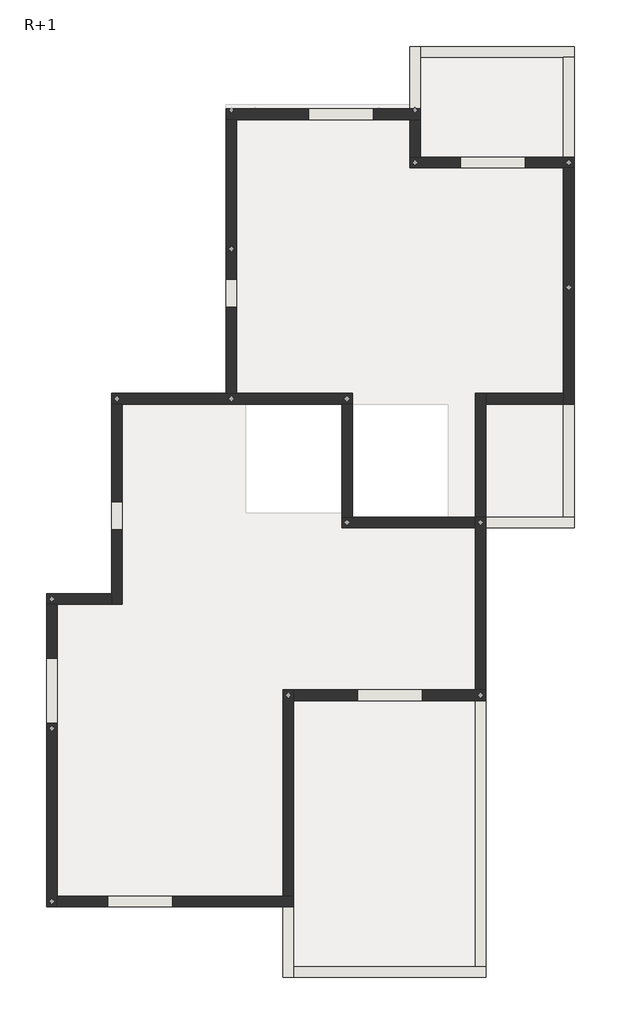
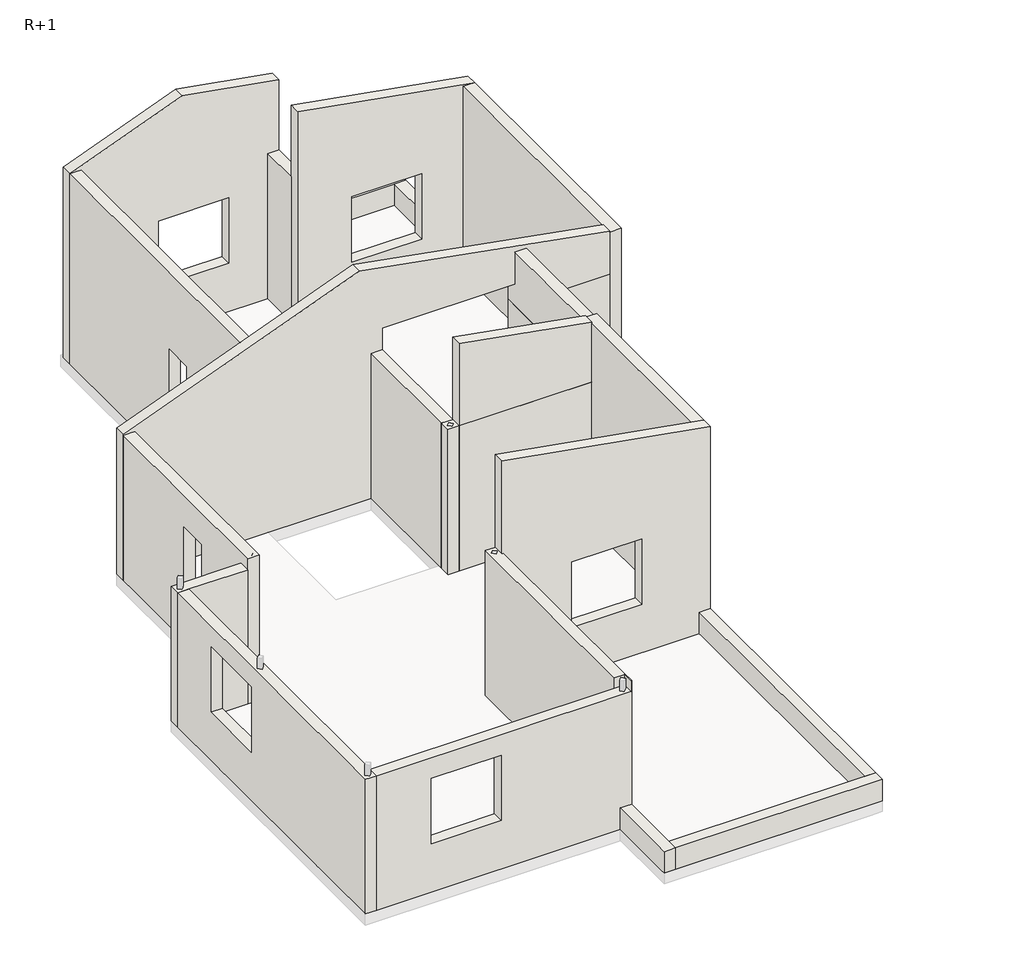
# One storey, part 1 of 2: 27 walls.
"""IFC4 building model written with IfcOpenShell, lengths in millimetres."""

from ifc_helpers import new_model, si_unit, frame, origin, place, context, project, spatial, polyline, outline, extrude, faceted_brep, element, save

model = new_model("IFC4")

# Units and contexts
model_context = context("Model", 3, world=origin())
ifc_project = project(units=[si_unit("LENGTHUNIT", "METRE", prefix="MILLI")], contexts=[model_context])

# Site, building, storey
site = spatial("IfcSite", under=ifc_project)
building = spatial("IfcBuilding", under=site)
storey = spatial("IfcBuildingStorey", under=building, Name="R+1", Elevation=2710.0)

# Walls
placement = place(None, origin())
element("IfcWall", 1, ObjectType="Bloc à brancher 20 cm", at=placement, inside=storey, context=model_context, shape_type="Brep", body=[
    faceted_brep([(834.5663791, 8348.2658581, 2710.0), (834.5663791, 9329.3149644, 2710.0), (834.5663791, 9529.3149644, 2710.0), (834.5663791, 9529.3149644, 3110.0), (834.5663791, 9329.3149644, 3110.0), (834.5663791, 8348.2658581, 3110.0), (634.5663791, 8348.2658581, 2710.0), (634.5663791, 8348.2658581, 3110.0), (634.5663791, 9529.3149644, 3110.0), (634.5663791, 9529.3149644, 2710.0), (763.1689261, 8348.2658581, 2710.0), (705.9638322, 8348.2658581, 2710.0)], [[[0, 1, 2, 3, 4, 5]], [[6, 7, 8, 9]], [[2, 1, 0, 10, 11, 6, 9]], [[5, 4, 3, 8, 7]], [[0, 5, 7, 6, 11, 10]], [[3, 2, 9, 8]]]),
])
element("IfcWall", 2, ObjectType="Bloc à brancher 20 cm", at=placement, inside=storey, context=model_context, shape_type="Brep", body=[
    faceted_brep([(834.5663791, 9329.3149644, 2710.0), (3544.5663998, 9329.3149644, 2710.0), (3744.5663998, 9329.3149644, 2710.0), (3744.5663998, 9329.3149644, 3110.0), (3544.5663998, 9329.3149644, 3110.0), (834.5663791, 9329.3149644, 3110.0), (834.5663791, 9529.3149644, 2710.0), (834.5663791, 9529.3149644, 3110.0), (3744.5663998, 9529.3149644, 3110.0), (3744.5663998, 9529.3149644, 2710.0)], [[[0, 1, 2, 3, 4, 5]], [[6, 7, 8, 9]], [[2, 1, 0, 6, 9]], [[5, 4, 3, 8, 7]], [[0, 5, 7, 6]], [[3, 2, 9, 8]]]),
])
element("IfcWall", 3, ObjectType="Bloc à brancher 20 cm", at=placement, inside=storey, context=model_context, shape_type="SweptSolid", body=[
    extrude(outline(polyline([(3544.5663998, 7432.979093), (3544.5663998, 9329.3149644), (3744.5663998, 9329.3149644), (3744.5663998, 7432.979093), (3544.5663998, 7432.979093)])), frame((0.0, 0.0, 2710.0), z_axis=(0.0, 0.0, 1.0), x_axis=(1.0, 0.0, 0.0)), (0.0, 0.0, 1.0), 400.0),
])
element("IfcWall", 4, ObjectType="Bloc à brancher 20 cm", at=placement, inside=storey, context=model_context, shape_type="Brep", body=[
    faceted_brep([(2074.5663639, 423.8353673, 2710.0), (3744.5663998, 423.8353673, 2710.0), (3744.5663998, 423.8353673, 3110.0), (2074.5663639, 423.8353673, 3110.0), (2074.5663639, 623.8353673, 2710.0), (2074.5663639, 623.8353673, 3110.0), (3544.5663998, 623.8353673, 3110.0), (3744.5663998, 623.8353673, 3110.0), (3744.5663998, 623.8353673, 2710.0), (3544.5663998, 623.8353673, 2710.0)], [[[0, 1, 2, 3]], [[4, 5, 6, 7, 8, 9]], [[1, 0, 4, 9, 8]], [[3, 2, 7, 6, 5]], [[0, 3, 5, 4]], [[2, 1, 8, 7]]]),
])
element("IfcWall", 5, ObjectType="Bloc à brancher 20 cm", at=placement, inside=storey, context=model_context, shape_type="SweptSolid", body=[
    extrude(outline(polyline([(3744.5663998, 2763.8353669), (3744.5663998, 623.8353673), (3544.5663998, 623.8353673), (3544.5663998, 2763.8353669), (3744.5663998, 2763.8353669)])), frame((0.0, 0.0, 2710.0), z_axis=(0.0, 0.0, 1.0), x_axis=(1.0, 0.0, 0.0)), (0.0, 0.0, 1.0), 400.0),
])
element("IfcWall", 6, ObjectType="Bloc à brancher 20 cm", at=placement, inside=storey, context=model_context, shape_type="Brep", body=[
    faceted_brep([(-1766.4904447, -6748.7020841, 2710.0), (-1766.4904447, -8086.16463, 2710.0), (-1766.4904447, -8086.16463, 3110.0), (-1766.4904447, -6748.7020841, 3110.0), (-1566.4904447, -6748.7020841, 2710.0), (-1566.4904447, -6748.7020841, 3110.0), (-1566.4904447, -7886.16463, 3110.0), (-1566.4904447, -8086.16463, 3110.0), (-1566.4904447, -8086.16463, 2710.0), (-1566.4904447, -7886.16463, 2710.0)], [[[0, 1, 2, 3]], [[4, 5, 6, 7, 8, 9]], [[1, 0, 4, 9, 8]], [[3, 2, 7, 6, 5]], [[0, 3, 5, 4]], [[2, 1, 8, 7]]]),
])
element("IfcWall", 7, ObjectType="Bloc à brancher 20 cm", at=placement, inside=storey, context=model_context, shape_type="Brep", body=[
    faceted_brep([(-1566.4904447, -8086.16463, 2710.0), (2074.5663809, -8086.16463, 2710.0), (2074.5663809, -8086.16463, 3110.0), (-1566.4904447, -8086.16463, 3110.0), (-1566.4904447, -7886.16463, 2710.0), (-1566.4904447, -7886.16463, 3110.0), (1874.5663809, -7886.16463, 3110.0), (2074.5663809, -7886.16463, 3110.0), (2074.5663809, -7886.16463, 2710.0), (1874.5663809, -7886.16463, 2710.0)], [[[0, 1, 2, 3]], [[4, 5, 6, 7, 8, 9]], [[1, 0, 4, 9, 8]], [[3, 2, 7, 6, 5]], [[0, 3, 5, 4]], [[2, 1, 8, 7]]]),
])
element("IfcWall", 8, ObjectType="Bloc à brancher 20 cm", at=placement, inside=storey, context=model_context, shape_type="SweptSolid", body=[
    extrude(outline(polyline([(2074.5663809, -2846.164631), (2074.5663809, -7886.16463), (1874.5663809, -7886.16463), (1874.5663809, -2846.164631), (2074.5663809, -2846.164631)])), frame((0.0, 0.0, 2710.0), z_axis=(0.0, 0.0, 1.0), x_axis=(1.0, 0.0, 0.0)), (0.0, 0.0, 1.0), 400.0),
])
element("IfcWall", 9, ObjectType="Parpaing 20cm", at=placement, inside=storey, context=model_context, shape_type="Brep", body=[
    faceted_brep([(-2645.4336004, 2963.8353669, 2710.0), (-2645.4336004, 8148.2658581, 2710.0), (-2645.4336004, 8148.2658581, 6251.7021272), (-2645.4336004, 2963.8353669, 6251.7021272), (-2645.4336004, 5124.1299225, 4825.0), (-2645.4336004, 5124.1299225, 3610.0), (-2645.4336004, 4594.1299225, 3610.0), (-2645.4336004, 4594.1299225, 4825.0), (-2845.4336004, 8148.2658581, 2710.0), (-2845.4336004, 2963.8353669, 2710.0), (-2845.4336004, 2963.8353669, 6251.7021272), (-2845.4336004, 8148.2658581, 6251.7021272), (-2845.4336004, 5124.1299225, 3610.0), (-2845.4336004, 5124.1299225, 4825.0), (-2845.4336004, 4594.1299225, 4825.0), (-2845.4336004, 4594.1299225, 3610.0), (-2745.4336004, 5751.8684051, 5410.0), (-2692.4005918, 5698.8353965, 5410.0), (-2745.4336004, 5645.8023879, 5410.0), (-2798.466609, 5698.8353965, 5410.0), (-2745.4336004, 5751.8684051, 2710.0), (-2692.4005918, 5698.8353965, 2710.0), (-2798.466609, 5698.8353965, 2710.0), (-2745.4336004, 5645.8023879, 2710.0)], [[[0, 1, 2, 3], [4, 5, 6, 7]], [[8, 9, 10, 11], [12, 13, 14, 15]], [[0, 3, 10, 9]], [[12, 5, 4, 13]], [[5, 12, 15, 6]], [[6, 15, 14, 7]], [[13, 4, 7, 14]], [[16, 17, 18, 19]], [[17, 16, 20, 21]], [[16, 19, 22, 20]], [[19, 18, 23, 22]], [[18, 17, 21, 23]], [[2, 1, 8, 11]], [[1, 0, 9, 8], [21, 20, 22, 23]], [[3, 2, 11, 10]]]),
])
element("IfcWall", 10, ObjectType="Parpaing 20cm", at=placement, inside=storey, context=model_context, shape_type="Brep", body=[
    faceted_brep([(-2845.4336004, 8148.2658581, 2710.0), (-2645.4336004, 8148.2658581, 2710.0), (634.5663791, 8148.2658581, 2710.0), (834.5663791, 8148.2658581, 2710.0), (834.5663791, 8148.2658581, 5410.0), (834.5663791, 8148.2658581, 6710.2441328), (-865.4336209, 8148.2658581, 7010.0), (-2845.4336004, 8148.2658581, 6251.7021272), (-2845.4336004, 8148.2658581, 5410.0), (-50.8307799, 8148.2658581, 4825.0), (-50.8307799, 8148.2658581, 3610.0), (-1280.8307799, 8148.2658581, 3610.0), (-1280.8307799, 8148.2658581, 4825.0), (834.5663791, 8348.2658581, 6710.2441328), (834.5663791, 8348.2658581, 3110.0), (834.5663791, 8348.2658581, 2710.0), (763.1689261, 8348.2658581, 2710.0), (763.1689261, 8348.2658581, 5410.0), (705.9638322, 8348.2658581, 5410.0), (705.9638322, 8348.2658581, 2710.0), (634.5663791, 8348.2658581, 2710.0), (-2716.8310535, 8348.2658581, 2710.0), (-2716.8310535, 8348.2658581, 5410.0), (-2774.0361474, 8348.2658581, 5410.0), (-2774.0361474, 8348.2658581, 2710.0), (-2845.4336004, 8348.2658581, 2710.0), (-2845.4336004, 8348.2658581, 5410.0), (-2845.4336004, 8348.2658581, 6251.7021272), (-865.4336209, 8348.2658581, 7010.0), (-50.8307799, 8348.2658581, 3610.0), (-50.8307799, 8348.2658581, 4825.0), (-1280.8307799, 8348.2658581, 4825.0), (-1280.8307799, 8348.2658581, 3610.0), (734.5663791, 8270.8023879, 5410.0), (681.5333706, 8323.8353965, 5410.0), (787.5993877, 8323.8353965, 5410.0), (787.5993877, 8323.8353965, 2710.0), (681.5333706, 8323.8353965, 2710.0), (734.5663791, 8270.8023879, 2710.0), (-2745.4336004, 8270.8023879, 5410.0), (-2798.466609, 8323.8353965, 5410.0), (-2692.4005918, 8323.8353965, 5410.0), (-2692.4005918, 8323.8353965, 2710.0), (-2798.466609, 8323.8353965, 2710.0), (-2745.4336004, 8270.8023879, 2710.0)], [[[0, 1, 2, 3, 4, 5, 6, 7, 8], [9, 10, 11, 12]], [[13, 14, 15, 16, 17, 18, 19, 20, 21, 22, 23, 24, 25, 26, 27, 28], [29, 30, 31, 32]], [[10, 9, 30, 29]], [[11, 10, 29, 32]], [[12, 11, 32, 31]], [[9, 12, 31, 30]], [[33, 34, 18, 17, 35]], [[36, 35, 17, 16]], [[34, 37, 19, 18]], [[34, 33, 38, 37]], [[33, 35, 36, 38]], [[39, 40, 23, 22, 41]], [[42, 41, 22, 21]], [[40, 43, 24, 23]], [[40, 39, 44, 43]], [[39, 41, 42, 44]], [[3, 2, 1, 0, 25, 24, 43, 44, 42, 21, 20, 19, 37, 38, 36, 16, 15]], [[6, 5, 13, 28]], [[7, 6, 28, 27]], [[15, 14, 13, 5, 4, 3]], [[0, 8, 7, 27, 26, 25]]]),
])
element("IfcWall", 11, ObjectType="Parpaing 20cm", at=placement, inside=storey, context=model_context, shape_type="SweptSolid", body=[
    extrude(outline(polyline([(634.5663791, 7432.979093), (634.5663791, 8148.2658581), (834.5663791, 8148.2658581), (834.5663791, 7432.979093), (634.5663791, 7432.979093)])), frame((0.0, 0.0, 2710.0), z_axis=(0.0, 0.0, 1.0), x_axis=(1.0, 0.0, 0.0)), (0.0, 0.0, 1.0), 2700.0),
])
element("IfcWall", 12, ObjectType="Parpaing 20cm", at=placement, inside=storey, context=model_context, shape_type="Brep", body=[
    faceted_brep([(634.5663791, 7232.979093, 2710.0), (3544.5663998, 7232.979093, 2710.0), (3744.5663998, 7232.979093, 2710.0), (3744.5663998, 7232.979093, 6197.1326153), (634.5663791, 7232.979093, 6745.5095289), (2819.1692225, 7232.979093, 4825.0), (2819.1692225, 7232.979093, 3610.0), (1589.1692225, 7232.979093, 3610.0), (1589.1692225, 7232.979093, 4825.0), (3744.5663998, 7432.979093, 2710.0), (3544.5663998, 7432.979093, 2710.0), (834.5663791, 7432.979093, 2710.0), (634.5663791, 7432.979093, 2710.0), (634.5663791, 7432.979093, 5410.0), (634.5663791, 7432.979093, 6745.5095289), (3744.5663998, 7432.979093, 6197.1326153), (3744.5663998, 7432.979093, 3110.0), (2819.1692225, 7432.979093, 3610.0), (2819.1692225, 7432.979093, 4825.0), (1589.1692225, 7432.979093, 4825.0), (1589.1692225, 7432.979093, 3610.0), (3644.5663998, 7386.0121016, 5410.0), (3697.5994084, 7332.979093, 5410.0), (3644.5663998, 7279.9460844, 5410.0), (3591.5333912, 7332.979093, 5410.0), (3644.5663998, 7386.0121016, 2710.0), (3697.5994084, 7332.979093, 2710.0), (3591.5333912, 7332.979093, 2710.0), (3644.5663998, 7279.9460844, 2710.0), (734.5663791, 7386.0121016, 5410.0), (787.5993877, 7332.979093, 5410.0), (734.5663791, 7279.9460844, 5410.0), (681.5333706, 7332.979093, 5410.0), (734.5663791, 7386.0121016, 2710.0), (787.5993877, 7332.979093, 2710.0), (681.5333706, 7332.979093, 2710.0), (734.5663791, 7279.9460844, 2710.0)], [[[0, 1, 2, 3, 4], [5, 6, 7, 8]], [[9, 10, 11, 12, 13, 14, 15, 16], [17, 18, 19, 20]], [[6, 5, 18, 17]], [[7, 6, 17, 20]], [[8, 7, 20, 19]], [[5, 8, 19, 18]], [[21, 22, 23, 24]], [[22, 21, 25, 26]], [[21, 24, 27, 25]], [[24, 23, 28, 27]], [[23, 22, 26, 28]], [[3, 2, 9, 16, 15]], [[0, 4, 14, 13, 12]], [[29, 30, 31, 32]], [[30, 29, 33, 34]], [[29, 32, 35, 33]], [[32, 31, 36, 35]], [[31, 30, 34, 36]], [[2, 1, 0, 12, 11, 10, 9], [26, 25, 27, 28], [34, 33, 35, 36]], [[4, 3, 15, 14]]]),
])
element("IfcWall", 13, ObjectType="Parpaing 20cm", at=placement, inside=storey, context=model_context, shape_type="Brep", body=[
    faceted_brep([(3544.5663998, 7232.979093, 2710.0), (3544.5663998, 2963.8353669, 2710.0), (3544.5663998, 2763.8353669, 2710.0), (3544.5663998, 2763.8353669, 5410.0), (3544.5663998, 2763.8353669, 6197.1326153), (3544.5663998, 7232.979093, 6197.1326153), (3744.5663998, 2763.8353669, 2710.0), (3744.5663998, 7232.979093, 2710.0), (3744.5663998, 7232.979093, 6197.1326153), (3744.5663998, 2763.8353669, 6197.1326153), (3644.5663998, 5026.0121016, 5410.0), (3697.5994084, 4972.979093, 5410.0), (3644.5663998, 4919.9460844, 5410.0), (3591.5333912, 4972.979093, 5410.0), (3644.5663998, 5026.0121016, 2710.0), (3697.5994084, 4972.979093, 2710.0), (3591.5333912, 4972.979093, 2710.0), (3644.5663998, 4919.9460844, 2710.0)], [[[0, 1, 2, 3, 4, 5]], [[6, 7, 8, 9]], [[0, 5, 8, 7]], [[10, 11, 12, 13]], [[11, 10, 14, 15]], [[10, 13, 16, 14]], [[13, 12, 17, 16]], [[12, 11, 15, 17]], [[2, 1, 0, 7, 6], [15, 14, 16, 17]], [[5, 4, 9, 8]], [[6, 9, 4, 3, 2]]]),
])
element("IfcWall", 14, ObjectType="Parpaing 20cm", at=placement, inside=storey, context=model_context, shape_type="Brep", body=[
    faceted_brep([(-455.4335965, 2963.8353669, 2710.0), (-2472.9274976, 2963.8353669, 2710.0), (-2645.4336004, 2963.8353669, 2710.0), (-2845.4336004, 2963.8353669, 2710.0), (-5012.6214092, 2963.8353669, 2710.0), (-5012.6214092, 2963.8353669, 5421.7152979), (-865.4336209, 2963.8353669, 7010.0), (3544.5663998, 2963.8353669, 6215.1562823), (3544.5663998, 2963.8353669, 5410.0), (2074.5663639, 2963.8353669, 5410.0), (2074.5663639, 2963.8353669, 5810.0), (1874.5663639, 2963.8353669, 5810.0), (-455.4335965, 2963.8353669, 5810.0), (-455.4335965, 2963.8353669, 5410.0), (-5012.6214092, 2763.8353669, 2710.0), (-4812.6214092, 2763.8353669, 2710.0), (-2472.9274976, 2763.8353669, 2710.0), (-655.4335965, 2763.8353669, 2710.0), (-455.4335965, 2763.8353669, 2710.0), (-455.4335965, 2763.8353669, 5410.0), (-455.4335965, 2763.8353669, 5810.0), (1874.5663639, 2763.8353669, 5810.0), (2074.5663639, 2763.8353669, 5810.0), (2074.5663639, 2763.8353669, 5410.0), (3544.5663998, 2763.8353669, 5410.0), (3544.5663998, 2763.8353669, 6197.1326153), (3544.5663998, 2763.8353669, 6215.1562823), (-865.4336209, 2763.8353669, 7010.0), (-5012.6214092, 2763.8353669, 5421.7152979), (-5012.6214092, 2763.8353669, 5410.0), (-4912.6214092, 2916.8683755, 5410.0), (-4859.5884006, 2863.8353669, 5410.0), (-4912.6214092, 2810.8023583, 5410.0), (-4965.6544178, 2863.8353669, 5410.0), (-4912.6214092, 2916.8683755, 2710.0), (-4859.5884006, 2863.8353669, 2710.0), (-4965.6544178, 2863.8353669, 2710.0), (-4912.6214092, 2810.8023583, 2710.0), (-2745.4336004, 2916.8683755, 5410.0), (-2692.4005918, 2863.8353669, 5410.0), (-2745.4336004, 2810.8023583, 5410.0), (-2798.466609, 2863.8353669, 5410.0), (-2745.4336004, 2916.8683755, 2710.0), (-2692.4005918, 2863.8353669, 2710.0), (-2798.466609, 2863.8353669, 2710.0), (-2745.4336004, 2810.8023583, 2710.0), (-502.4005879, 2863.8353669, 2710.0), (-555.4335965, 2916.8683755, 2710.0), (-608.4666051, 2863.8353669, 2710.0), (-555.4335965, 2810.8023583, 2710.0), (-455.4335965, 2764.0588408, 5810.0), (-555.4335965, 2916.8683755, 5410.0), (-502.4005879, 2863.8353669, 5410.0), (-555.4335965, 2810.8023583, 5410.0), (-608.4666051, 2863.8353669, 5410.0)], [[[0, 1, 2, 3, 4, 5, 6, 7, 8, 9, 10, 11, 12, 13]], [[14, 15, 16, 17, 18, 19, 20, 21, 22, 23, 24, 25, 26, 27, 28, 29]], [[5, 4, 14, 29, 28]], [[30, 31, 32, 33]], [[31, 30, 34, 35]], [[30, 33, 36, 34]], [[33, 32, 37, 36]], [[32, 31, 35, 37]], [[38, 39, 40, 41]], [[39, 38, 42, 43]], [[38, 41, 44, 42]], [[41, 40, 45, 44]], [[40, 39, 43, 45]], [[4, 3, 2, 1, 0, 18, 17, 16, 15, 14], [43, 42, 44, 45], [35, 34, 36, 37], [46, 47, 48, 49]], [[6, 5, 28, 27]], [[7, 6, 27, 26]], [[12, 11, 10, 22, 21, 20, 50]], [[51, 52, 53, 54]], [[52, 51, 47, 46]], [[51, 54, 48, 47]], [[54, 53, 49, 48]], [[53, 52, 46, 49]], [[0, 13, 12, 50, 20, 19, 18]], [[9, 8, 24, 23]], [[8, 7, 26, 25, 24]], [[10, 9, 23, 22]]]),
])
element("IfcWall", 15, ObjectType="Parpaing 20cm", at=placement, inside=storey, context=model_context, shape_type="Brep", body=[
    faceted_brep([(-5012.6214092, 2763.8353669, 2710.0), (-5012.6214092, -828.5605356, 2710.0), (-5012.6214092, -1028.5605356, 2710.0), (-5012.6214092, -1028.5605356, 5210.0), (-5012.6214092, -1028.5605356, 5410.0), (-5012.6214092, 2763.8353669, 5410.0), (-5012.6214092, 916.6629583, 4825.0), (-5012.6214092, 386.6629583, 4825.0), (-5012.6214092, 386.6629583, 3610.0), (-5012.6214092, 916.6629583, 3610.0), (-4812.6214092, 2763.8353669, 2710.0), (-4812.6214092, 2763.8353669, 5410.0), (-4812.6214092, -1028.5605356, 5410.0), (-4812.6214092, -1028.5605356, 2710.0), (-4812.6214092, 916.6629583, 4825.0), (-4812.6214092, 916.6629583, 3610.0), (-4812.6214092, 386.6629583, 3610.0), (-4812.6214092, 386.6629583, 4825.0)], [[[0, 1, 2, 3, 4, 5], [6, 7, 8, 9]], [[10, 11, 12, 13], [14, 15, 16, 17]], [[2, 1, 0, 10, 13]], [[5, 4, 12, 11]], [[0, 5, 11, 10]], [[4, 3, 2, 13, 12]], [[15, 14, 6, 9]], [[16, 15, 9, 8]], [[17, 16, 8, 7]], [[14, 17, 7, 6]]]),
])
element("IfcWall", 16, ObjectType="Parpaing 20cm", at=placement, inside=storey, context=model_context, shape_type="Brep", body=[
    faceted_brep([(-5012.6214092, -828.5605356, 2710.0), (-6246.4904447, -828.5605356, 2710.0), (-6246.4904447, -828.5605356, 5210.0), (-5012.6214092, -828.5605356, 5210.0), (-6246.4904447, -1028.5605356, 2710.0), (-6046.4904447, -1028.5605356, 2710.0), (-5012.6214092, -1028.5605356, 2710.0), (-5012.6214092, -1028.5605356, 5210.0), (-6046.4904447, -1028.5605356, 5210.0), (-6246.4904447, -1028.5605356, 5210.0), (-6093.4574361, -928.5605356, 2710.0), (-6146.4904447, -875.527527, 2710.0), (-6199.5234533, -928.5605356, 2710.0), (-6146.4904447, -981.5935442, 2710.0), (-6093.4574361, -928.5605356, 5210.0), (-6146.4904447, -875.527527, 5210.0), (-6199.5234533, -928.5605356, 5210.0), (-6146.4904447, -981.5935442, 5210.0)], [[[0, 1, 2, 3]], [[4, 5, 6, 7, 8, 9]], [[1, 0, 6, 5, 4], [10, 11, 12, 13]], [[6, 0, 3, 7]], [[1, 4, 9, 2]], [[11, 10, 14, 15]], [[12, 11, 15, 16]], [[13, 12, 16, 17]], [[10, 13, 17, 14]], [[3, 2, 9, 8, 7], [15, 14, 17, 16]]]),
])
element("IfcWall", 17, ObjectType="Parpaing 20cm", at=placement, inside=storey, context=model_context, shape_type="Brep", body=[
    faceted_brep([(-6246.4904447, -1028.5605356, 2710.0), (-6246.4904447, -6748.7020841, 2710.0), (-6246.4904447, -6748.7020841, 5210.0), (-6246.4904447, -1028.5605356, 5210.0), (-6246.4904447, -2045.9447999, 3610.0), (-6246.4904447, -2045.9447999, 4825.0), (-6246.4904447, -3275.9447999, 4825.0), (-6246.4904447, -3275.9447999, 3610.0), (-6046.4904447, -6748.7020841, 2710.0), (-6046.4904447, -6548.7020841, 2710.0), (-6046.4904447, -1028.5605356, 2710.0), (-6046.4904447, -1028.5605356, 5210.0), (-6046.4904447, -6548.7020841, 5210.0), (-6046.4904447, -6748.7020841, 5210.0), (-6046.4904447, -2045.9447999, 4825.0), (-6046.4904447, -2045.9447999, 3610.0), (-6046.4904447, -3275.9447999, 3610.0), (-6046.4904447, -3275.9447999, 4825.0), (-6093.4574361, -3373.5605356, 2710.0), (-6146.4904447, -3320.527527, 2710.0), (-6199.5234533, -3373.5605356, 2710.0), (-6146.4904447, -3426.5935442, 2710.0), (-6093.4574361, -6648.7020841, 2710.0), (-6146.4904447, -6595.6690755, 2710.0), (-6199.5234533, -6648.7020841, 2710.0), (-6146.4904447, -6701.7350927, 2710.0), (-6093.4574361, -3373.5605356, 5210.0), (-6146.4904447, -3320.527527, 5210.0), (-6199.5234533, -3373.5605356, 5210.0), (-6146.4904447, -3426.5935442, 5210.0), (-6093.4574361, -6648.7020841, 5210.0), (-6146.4904447, -6595.6690755, 5210.0), (-6199.5234533, -6648.7020841, 5210.0), (-6146.4904447, -6701.7350927, 5210.0)], [[[0, 1, 2, 3], [4, 5, 6, 7]], [[8, 9, 10, 11, 12, 13], [14, 15, 16, 17]], [[1, 0, 10, 9, 8], [18, 19, 20, 21], [22, 23, 24, 25]], [[10, 0, 3, 11]], [[1, 8, 13, 2]], [[15, 14, 5, 4]], [[16, 15, 4, 7]], [[17, 16, 7, 6]], [[14, 17, 6, 5]], [[19, 18, 26, 27]], [[20, 19, 27, 28]], [[21, 20, 28, 29]], [[18, 21, 29, 26]], [[23, 22, 30, 31]], [[24, 23, 31, 32]], [[25, 24, 32, 33]], [[22, 25, 33, 30]], [[3, 2, 13, 12, 11], [31, 30, 33, 32], [27, 26, 29, 28]]]),
])
element("IfcWall", 18, ObjectType="Parpaing 20cm", at=placement, inside=storey, context=model_context, shape_type="Brep", body=[
    faceted_brep([(-6046.4904447, -6748.7020841, 2710.0), (-1766.4904447, -6748.7020841, 2710.0), (-1566.4904447, -6748.7020841, 2710.0), (-1566.4904447, -6748.7020841, 3110.0), (-1566.4904447, -6748.7020841, 5410.0), (-1572.6214092, -6748.7020841, 5410.0), (-1572.6214092, -6748.7020841, 5210.0), (-6046.4904447, -6748.7020841, 5210.0), (-3861.3591936, -6748.7020841, 4825.0), (-3861.3591936, -6748.7020841, 3610.0), (-5091.3591936, -6748.7020841, 3610.0), (-5091.3591936, -6748.7020841, 4825.0), (-1566.4904447, -6548.7020841, 2710.0), (-1766.4904447, -6548.7020841, 2710.0), (-6046.4904447, -6548.7020841, 2710.0), (-6046.4904447, -6548.7020841, 5210.0), (-1572.6214092, -6548.7020841, 5210.0), (-1572.6214092, -6548.7020841, 5410.0), (-1566.4904447, -6548.7020841, 5410.0), (-3861.3591936, -6548.7020841, 3610.0), (-3861.3591936, -6548.7020841, 4825.0), (-5091.3591936, -6548.7020841, 4825.0), (-5091.3591936, -6548.7020841, 3610.0)], [[[0, 1, 2, 3, 4, 5, 6, 7], [8, 9, 10, 11]], [[12, 13, 14, 15, 16, 17, 18], [19, 20, 21, 22]], [[2, 1, 0, 14, 13, 12]], [[4, 18, 17, 5]], [[14, 0, 7, 15]], [[9, 8, 20, 19]], [[10, 9, 19, 22]], [[11, 10, 22, 21]], [[8, 11, 21, 20]], [[6, 16, 15, 7]], [[16, 6, 5, 17]], [[2, 12, 18, 4, 3]]]),
])
element("IfcWall", 19, ObjectType="Parpaing 20cm", at=placement, inside=storey, context=model_context, shape_type="Brep", body=[
    faceted_brep([(-1566.4904447, -6548.7020841, 2710.0), (-1566.4904447, -2846.164631, 2710.0), (-1566.4904447, -2646.164631, 2710.0), (-1566.4904447, -2646.164631, 5410.0), (-1566.4904447, -2846.164631, 5410.0), (-1566.4904447, -6548.7020841, 5410.0), (-1766.4904447, -2646.164631, 2710.0), (-1766.4904447, -6548.7020841, 2710.0), (-1766.4904447, -6548.7020841, 5410.0), (-1766.4904447, -2646.164631, 5410.0), (-1613.4574361, -2746.164631, 2710.0), (-1666.4904447, -2693.1316224, 2710.0), (-1719.5234533, -2746.164631, 2710.0), (-1666.4904447, -2799.1976396, 2710.0), (-1593.4574361, -2646.164631, 5410.0), (-1572.6214092, -6548.7020841, 5410.0), (-1666.4904447, -2693.1316224, 5410.0), (-1613.4574361, -2746.164631, 5410.0), (-1666.4904447, -2799.1976396, 5410.0), (-1719.5234533, -2746.164631, 5410.0)], [[[0, 1, 2, 3, 4, 5]], [[6, 7, 8, 9]], [[2, 1, 0, 7, 6], [10, 11, 12, 13]], [[5, 4, 3, 14, 9, 8, 15], [16, 17, 18, 19]], [[5, 15, 8, 7, 0]], [[10, 17, 16, 11]], [[11, 16, 19, 12]], [[12, 19, 18, 13]], [[17, 10, 13, 18]], [[3, 2, 6, 9, 14]]]),
])
element("IfcWall", 20, ObjectType="Parpaing 20cm", at=placement, inside=storey, context=model_context, shape_type="Brep", body=[
    faceted_brep([(-1566.4904447, -2846.164631, 2710.0), (1874.5663809, -2846.164631, 2710.0), (2074.5663639, -2846.164631, 2710.0), (2074.5663639, -2846.164631, 3110.0), (2074.5663639, -2846.164631, 6491.7283134), (-1593.4574361, -2846.164631, 7133.7448671), (-1593.4574361, -2846.164631, 5410.0), (-1566.4904447, -2846.164631, 5410.0), (869.1692225, -2846.164631, 4825.0), (869.1692225, -2846.164631, 3610.0), (-360.8307775, -2846.164631, 3610.0), (-360.8307775, -2846.164631, 4825.0), (2074.5663639, -2646.164631, 2710.0), (1874.5663639, -2646.164631, 2710.0), (-1566.4904447, -2646.164631, 2710.0), (-1566.4904447, -2646.164631, 5410.0), (-1593.4574361, -2646.164631, 5410.0), (-1593.4574361, -2646.164631, 5900.0), (-1593.4574361, -2646.164631, 7133.7448671), (2074.5663639, -2646.164631, 6491.7283134), (869.1692225, -2646.164631, 3610.0), (869.1692225, -2646.164631, 4825.0), (-360.8307775, -2646.164631, 4825.0), (-360.8307775, -2646.164631, 3610.0), (1974.5663639, -2693.1316224, 5410.0), (2027.5993725, -2746.164631, 5410.0), (1974.5663639, -2799.1976396, 5410.0), (1921.5333553, -2746.164631, 5410.0), (1974.5663639, -2693.1316224, 2710.0), (2027.5993725, -2746.164631, 2710.0), (1921.5333553, -2746.164631, 2710.0), (1974.5663639, -2799.1976396, 2710.0)], [[[0, 1, 2, 3, 4, 5, 6, 7], [8, 9, 10, 11]], [[12, 13, 14, 15, 16, 17, 18, 19], [20, 21, 22, 23]], [[9, 8, 21, 20]], [[10, 9, 20, 23]], [[11, 10, 23, 22]], [[8, 11, 22, 21]], [[24, 25, 26, 27]], [[25, 24, 28, 29]], [[24, 27, 30, 28]], [[27, 26, 31, 30]], [[26, 25, 29, 31]], [[4, 3, 2, 12, 19]], [[2, 1, 0, 14, 13, 12], [29, 28, 30, 31]], [[5, 4, 19, 18]], [[16, 15, 7, 6]], [[0, 7, 15, 14]], [[6, 5, 18, 17, 16]]]),
])
element("IfcWall", 21, ObjectType="Parpaing 20cm", at=placement, inside=storey, context=model_context, shape_type="Brep", body=[
    faceted_brep([(2074.5663639, -2646.164631, 2710.0), (2074.5663639, 423.8353673, 2710.0), (2074.5663639, 623.8353673, 2710.0), (2074.5663639, 623.8353673, 3110.0), (2074.5663639, 623.8353673, 5410.0), (2074.5663639, 623.8353673, 6410.0), (2074.5663639, 623.8353673, 6491.7283134), (2074.5663639, -2646.164631, 6491.7283134), (1874.5663639, 623.8353673, 2710.0), (1874.5663639, 423.8353673, 2710.0), (1874.5663639, -2646.164631, 2710.0), (1874.5663639, -2646.164631, 6491.7283134), (1874.5663639, 623.8353673, 6491.7283134), (1874.5663639, 623.8353673, 6410.0), (1874.5663639, 623.8353673, 5410.0), (1974.5663639, 576.8683759, 5410.0), (2027.5993725, 523.8353673, 5410.0), (1974.5663639, 470.8023588, 5410.0), (1921.5333553, 523.8353673, 5410.0), (1974.5663639, 576.8683759, 2710.0), (2027.5993725, 523.8353673, 2710.0), (1921.5333553, 523.8353673, 2710.0), (1974.5663639, 470.8023588, 2710.0)], [[[0, 1, 2, 3, 4, 5, 6, 7]], [[8, 9, 10, 11, 12, 13, 14]], [[15, 16, 17, 18]], [[16, 15, 19, 20]], [[15, 18, 21, 19]], [[18, 17, 22, 21]], [[17, 16, 20, 22]], [[0, 7, 11, 10]], [[2, 1, 0, 10, 9, 8], [20, 19, 21, 22]], [[7, 6, 12, 11]], [[8, 14, 13, 12, 6, 5, 4, 3, 2]]]),
])
element("IfcWall", 22, ObjectType="Parpaing 20cm", at=placement, inside=storey, context=model_context, shape_type="Brep", body=[
    faceted_brep([(1874.5663639, 623.8353673, 2710.0), (-455.4335965, 623.8353673, 2710.0), (-655.4335965, 623.8353673, 2710.0), (-655.4335965, 623.8353673, 5410.0), (-455.4335965, 623.8353673, 5410.0), (1874.5663639, 623.8353673, 5410.0), (-655.4335965, 423.8353673, 2710.0), (1874.5663639, 423.8353673, 2710.0), (1874.5663639, 423.8353673, 5410.0), (-655.4335965, 423.8353673, 5410.0), (-502.4005879, 523.8353673, 2710.0), (-555.4335965, 576.8683759, 2710.0), (-608.4666051, 523.8353673, 2710.0), (-555.4335965, 470.8023588, 2710.0), (-555.4335965, 576.8683759, 5410.0), (-502.4005879, 523.8353673, 5410.0), (-555.4335965, 470.8023588, 5410.0), (-608.4666051, 523.8353673, 5410.0)], [[[0, 1, 2, 3, 4, 5]], [[6, 7, 8, 9]], [[2, 1, 0, 7, 6], [10, 11, 12, 13]], [[5, 4, 3, 9, 8], [14, 15, 16, 17]], [[3, 2, 6, 9]], [[5, 8, 7, 0]], [[10, 15, 14, 11]], [[11, 14, 17, 12]], [[12, 17, 16, 13]], [[15, 10, 13, 16]]]),
])
element("IfcWall", 23, ObjectType="Parpaing 20cm", at=placement, inside=storey, context=model_context, shape_type="SweptSolid", body=[
    extrude(outline(polyline([(-455.4335965, 2763.8353669), (-455.4335965, 623.8353673), (-655.4335965, 623.8353673), (-655.4335965, 2763.8353669), (-455.4335965, 2763.8353669)])), frame((0.0, 0.0, 2710.0), z_axis=(0.0, 0.0, 1.0), x_axis=(1.0, 0.0, 0.0)), (0.0, 0.0, 1.0), 2700.0),
])
element("IfcWall", 24, ObjectType="Parpaing 20cm", at=placement, inside=storey, context=model_context, shape_type="Brep", body=[
    faceted_brep([(1874.5663639, 2963.8353669, 2710.0), (1874.5663639, 623.8353673, 2710.0), (1874.5663639, 623.8353673, 5410.0), (1874.5663639, 2963.8353669, 5410.0), (2074.5663639, 2963.8353669, 2710.0), (2074.5663639, 2963.8353669, 5410.0), (2074.5663639, 2763.8353669, 5410.0), (2074.5663639, 623.8353673, 5410.0), (2074.5663639, 623.8353673, 2710.0), (2074.5663639, 2763.8353669, 2710.0)], [[[0, 1, 2, 3]], [[4, 5, 6, 7, 8, 9]], [[1, 0, 4, 9, 8]], [[3, 2, 7, 6, 5]], [[0, 3, 5, 4]], [[1, 8, 7, 2]]]),
])
element("IfcWall", 25, ObjectType="Parpaing 20cm", at=placement, inside=storey, context=model_context, shape_type="Brep", body=[
    faceted_brep([(-455.4335965, 423.8353673, 2710.0), (1874.5663639, 423.8353673, 2710.0), (1874.5663639, 423.8353673, 6526.8640755), (-455.4335965, 423.8353673, 6937.7059336), (-455.4335965, 623.8353673, 2710.0), (-455.4335965, 623.8353673, 6937.7059336), (1874.5663639, 623.8353673, 6526.8640755), (1874.5663639, 623.8353673, 6491.7283134), (1874.5663639, 623.8353673, 2710.0)], [[[0, 1, 2, 3]], [[4, 5, 6, 7, 8]], [[0, 3, 5, 4]], [[1, 0, 4, 8]], [[3, 2, 6, 5]], [[1, 8, 7, 6, 2]]]),
])
element("IfcWall", 26, ObjectType="Parpaing 20cm", at=placement, inside=storey, context=model_context, shape_type="Brep", body=[
    faceted_brep([(2074.5663639, 623.8353673, 2710.0), (2074.5663639, 2763.8353669, 2710.0), (2074.5663639, 2963.8353669, 2710.0), (2074.5663639, 2963.8353669, 5410.0), (2074.5663639, 2963.8353669, 5810.0), (2074.5663639, 2763.8353669, 5810.0), (2074.5663639, 2763.8353669, 6410.0), (2074.5663639, 623.8353673, 6410.0), (1874.5663639, 2963.8353669, 2710.0), (1874.5663639, 623.8353673, 2710.0), (1874.5663639, 623.8353673, 6410.0), (1874.5663639, 2763.8353669, 6410.0), (1874.5663639, 2763.8353669, 5810.0), (1874.5663639, 2764.0588408, 5810.0), (1874.5663639, 2963.8353669, 5810.0), (1874.5663639, 2963.8353669, 5410.0), (1974.5663639, 2916.8683755, 5410.0), (2027.5993725, 2863.8353669, 5410.0), (1974.5663639, 2810.8023583, 5410.0), (1921.5333553, 2863.8353669, 5410.0), (1974.5663639, 2916.8683755, 2710.0), (2027.5993725, 2863.8353669, 2710.0), (1921.5333553, 2863.8353669, 2710.0), (1974.5663639, 2810.8023583, 2710.0), (2074.1692225, 2963.8353669, 5810.0)], [[[0, 1, 2, 3, 4, 5, 6, 7]], [[8, 9, 10, 11, 12, 13, 14, 15]], [[16, 17, 18, 19]], [[17, 16, 20, 21]], [[16, 19, 22, 20]], [[19, 18, 23, 22]], [[18, 17, 21, 23]], [[2, 1, 0, 9, 8], [21, 20, 22, 23]], [[7, 6, 11, 10]], [[0, 7, 10, 9]], [[5, 4, 24, 14, 13, 12]], [[2, 8, 15, 14, 24, 4, 3]], [[11, 6, 5, 12]]]),
])
element("IfcWall", 27, ObjectType="Parpaing 20cm", at=placement, inside=storey, context=model_context, shape_type="SweptSolid", body=[
    extrude(outline(polyline([(3544.5663998, 2763.8353669), (2074.5663639, 2763.8353669), (2074.5663639, 2963.8353669), (3544.5663998, 2963.8353669), (3544.5663998, 2763.8353669)])), frame((0.0, 0.0, 2710.0), z_axis=(0.0, 0.0, 1.0), x_axis=(1.0, 0.0, 0.0)), (0.0, 0.0, 1.0), 2700.0),
])

save(model, "model.ifc")

# Revit data of these elements
# Type "Bloc à brancher 20 cm"
#   Layers, outside or top first: 0.025 m "Blocs béton manufacturés" (function 1); 0.150 m "Béton - Coulé sur place - Béton25" (function 1); 0.025 m "Blocs béton manufacturés" (function 1)
# Type "Parpaing 20cm"
#   Layers, outside or top first: 0.200 m "Brique, commune" (function 1)
# Elements 1, 2, 4, 6, 7 (IfcWall, "Bloc à brancher 20 cm")
#   Top Offset = 0.000 m
#   Base Offset = 0.000 m
#   wall height = 0.400 m
#   Phase Created = Nouvelle construction
#   Base Constraint = R+1
#   Top Constraint = As acrotère R+1
#   Materials on its faces: "Blocs béton manufacturés", "Mur par défaut"
# Elements 3, 5, 8 (IfcWall, "Bloc à brancher 20 cm")
#   Top Offset = 0.000 m
#   Base Offset = 0.000 m
#   wall height = 0.400 m
#   Phase Created = Nouvelle construction
#   Base Constraint = R+1
#   Top Constraint = As acrotère R+1
#   Materials on its faces: "Mur par défaut", "Blocs béton manufacturés"
# Elements 9, 10, 11, 12, 13, 14, 15, 16, 17, 18, 19, 20, 21, 22, 23, 24, 25, 26, 27 (IfcWall, "Parpaing 20cm")
#   Comments = ""
#   Top Offset = 0.000 m
#   Base Offset = 0.000 m
#   wall height = 2.700 m
#   Phase Created = Nouvelle construction
#   Base Constraint = R+1
#   Top Constraint = Toiture brut
#   Materials on its faces: "Brique, commune"
# Materials
#   "Blocs béton manufacturés": class "Maçonnerie", colour RGB 152 154 138, transparency 0, Description = "Blocs béton manufacturés", Cost = 0
#   "Béton - Coulé sur place - Béton25": class "Béton", colour RGB 192 192 192, transparency 0, Cost = 0
#   "Brique, commune": class "Maçonnerie", colour RGB 85 47 55, transparency 0, Description = "Brique commune", Cost = 0
#   "Mur par défaut": class "Divers", colour RGB 128 128 128, transparency 0, Cost = 0
